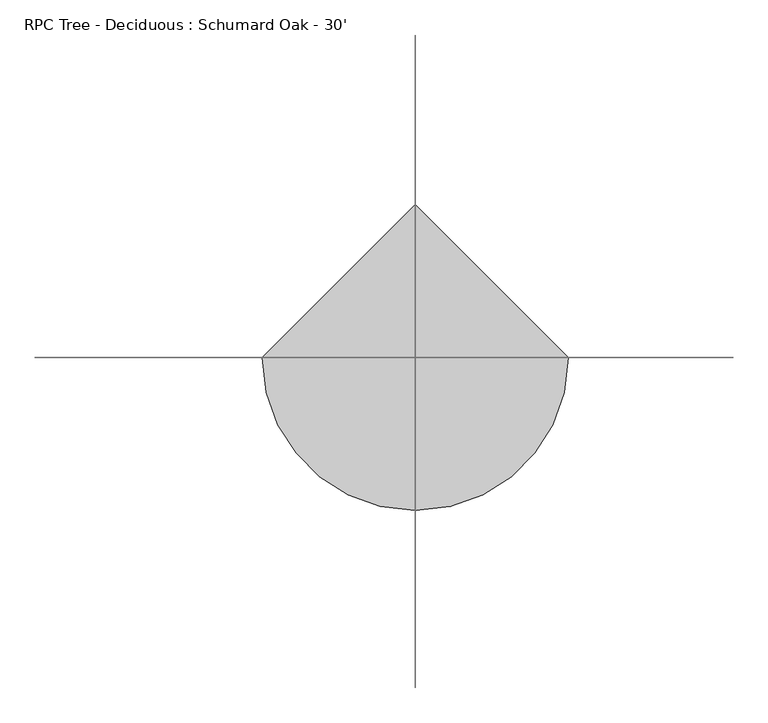
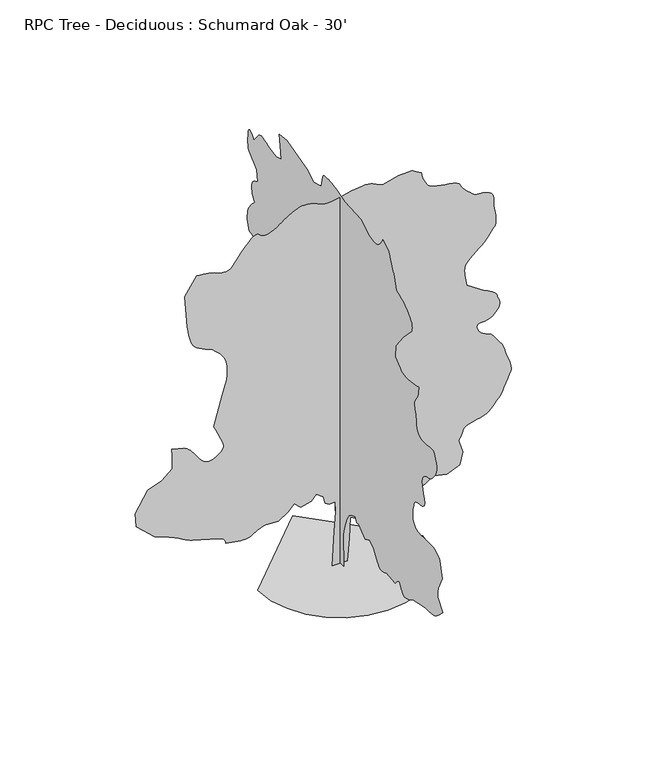
# IFC4 building model written with IfcOpenShell, lengths in millimetres: geographic element geometry, RPC Tree - Deciduous : Schumard Oak - 30'.
# Revit data of these elements (continued)
# Type "RPC Tree - Deciduous : Schumard Oak - 30'" (continued)
#   built-in parameter 1005198 = "{2, 15},{39, RPC-16-FXGQ-AS80-PNHH-0000-ST1L-LVER-AU},{1, 0},{1, 0},{2, 13},{1, 8},{5, Color},{1, 0},{1, 0},{3, 0.8},{3, 0.8},{3, 0.8},{1, 8},{7, BBoxMin},{1, 0},{1, 0},{1, 0},{1, 0},{1, 0},{1, 8},{7, BBoxMax},{1, 0},{1, 0},{1, 0},{1, 0},{1, 0},{2, 11},{9, RPCTypeId},{1, 0},{1, 0},{39, RPC-16-FXGQ-AS80-PNHH-0000-ST1L-LVER-AU},{1, 6},{14, RPCPlantHeight},{1, 0},{1, 0},{2, 30},{2, 11},{7, keyword},{1, 0},{1, 0},{34, :RPCs:Trees [General]:Geometry:RPC},{2, 11},{8, category},{1, 0},{1, 0},{15, Trees [General]},{2, 11},{12, LocalizedUID},{1, 0},{1, 0},{11, Shumard Oak},{2, 14},{6, Height},{1, 0},{1, 0},{2, 30},{1, 2},{16, Cast Reflections},{1, 0},{1, 0},{1, 0},{1, 2},{12, Cast Shadows},{1, 0},{1, 0},{1, 1},{1, 2},{9, Lock View},{1, 0},{1, 0},{1, 0},{1, 4},{5, ViewC},{1, 0},{1, 0},{1, 0},{21, assetlibrary_base.fbx},{1, 5},"
#   built-in parameter 1005195 = "RPC-16-FXGQ-AS80-PNHH-0000-ST1L-LVER-AU"
#   Type Comments = "Schumard Oak"
#   Assembly Code = "G2050500"
#   Height = 30' - 0"
#   Default Elevation = 0
